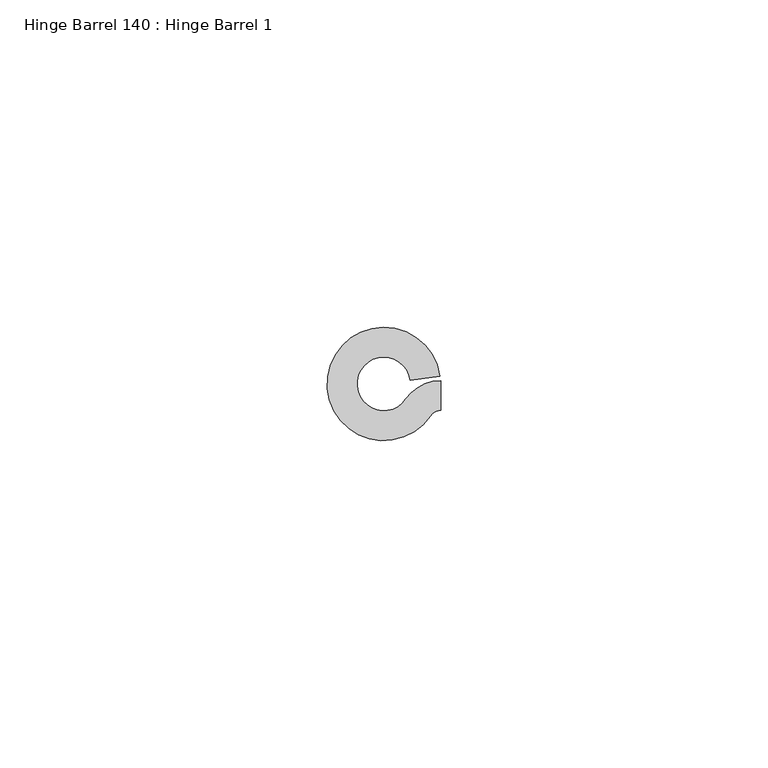
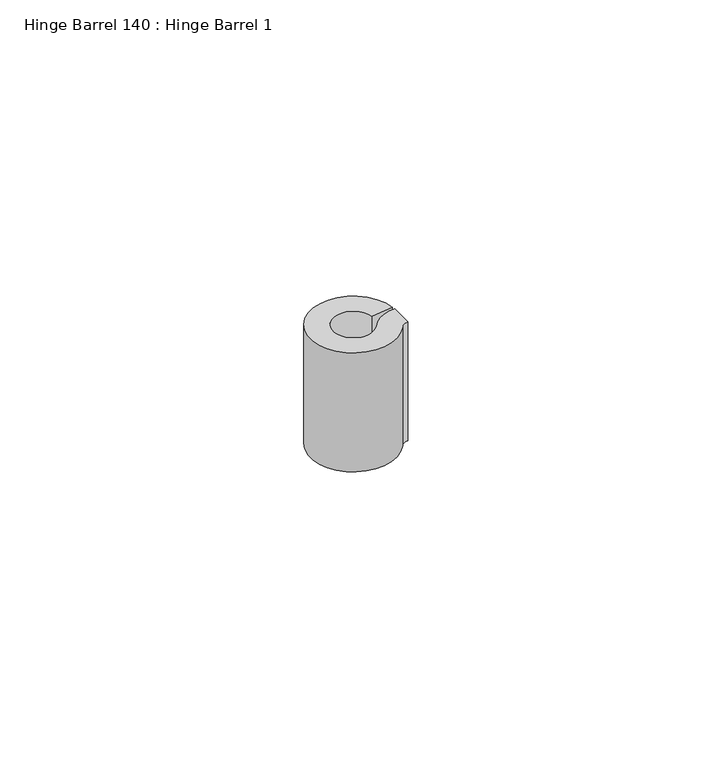
"""IFC4 building model written with IfcOpenShell, lengths in millimetres: proxy geometry, Hinge Barrel 140 : Hinge Barrel 1."""

from ifc_helpers import new_model, si_unit, point, frame, frame_2d, origin, place, context, project, spatial, polyline, circle_curve, trimmed, segment, composite_curve, outline, extrude, source, transform, mapped, element, save


def hinge_barrel_140_hinge_barrel_1_53ebecfd(model_context):
    return source(origin(), model_context, "Body", "SweptSolid", [
        extrude(outline(composite_curve([segment(trimmed(circle_curve(frame_2d((587327.8245257, -536316.2443067)), 6.4044851), [point((587322.5194669, -536312.6563017))], [point((587327.8245257, -536309.8398216))], False, "CARTESIAN"), True, "CONTINUOUS"), segment(polyline([(587327.8245257, -536309.8398216), (587327.8245257, -536314.4038841)]), True, "CONTINUOUS"), segment(trimmed(circle_curve(frame_2d((587327.8245257, -536316.2443067)), 1.8404226), [point((587327.8245257, -536314.4038841))], [point((587326.3000393, -536315.2132409))], True, "CARTESIAN"), True, "CONTINUOUS"), segment(trimmed(circle_curve(frame_2d((587319.1320739, -536310.3652841)), 8.6534625), [point((587326.3000393, -536315.2132409))], [point((587327.7022899, -536309.1678654))], False, "CARTESIAN"), True, "CONTINUOUS"), segment(polyline([(587327.7022899, -536309.1678654), (587323.1821338, -536309.7994153)]), True, "CONTINUOUS"), segment(trimmed(circle_curve(frame_2d((587319.1320739, -536310.3652841)), 4.0894), [point((587323.1821338, -536309.7994153))], [point((587322.5194669, -536312.6563017))], True, "CARTESIAN"), True, "CONTINUOUS")], self_intersect=False)), frame((0.0, 0.0, 1149.35), z_axis=(0.0, 0.0, 1.0), x_axis=(1.0, 0.0, 0.0)), (0.0, 0.0, 1.0), 25.4),
    ])


if __name__ == "__main__":
    model = new_model("IFC4")
    model_context = context("Model", 3, world=origin())
    ifc_project = project(units=[si_unit("LENGTHUNIT", "METRE", prefix="MILLI")], contexts=[model_context])
    site = spatial("IfcSite", under=ifc_project)
    building = spatial("IfcBuilding", under=site)
    placement = place(None, origin())
    hinge_barrel_140_hinge_barrel_1_shape = hinge_barrel_140_hinge_barrel_1_53ebecfd(model_context)
    element("IfcBuildingElementProxy", 1, Name="Hinge Barrel 140 : Hinge Barrel 1", ObjectType="Hinge Barrel 140 : Hinge Barrel 1", at=placement, inside=building, context=model_context, shape_type="MappedRepresentation", body=[
        mapped(hinge_barrel_140_hinge_barrel_1_shape, transform((0.0, 0.0, 0.0), x_axis=(1.0, 0.0, 0.0), y_axis=(0.0, 1.0, 0.0), z_axis=(0.0, 0.0, 1.0))),
    ])
    save(model, "model.ifc")

# Revit data of these elements
# Element 1 (IfcBuildingElementProxy, "Hinge Barrel 140 : Hinge Barrel 1")
#   Materials on its faces: "6\"X6\" WELD-ON STL BUTT HINGE"
# Materials
#   "6\"X6\" WELD-ON STL BUTT HINGE": class "Metal", colour RGB 189 187 185, transparency 0, Description = "Carbon steel", Cost = 0
